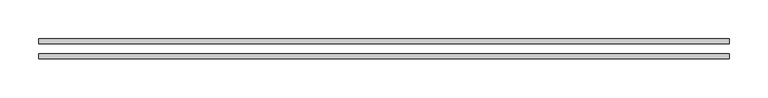
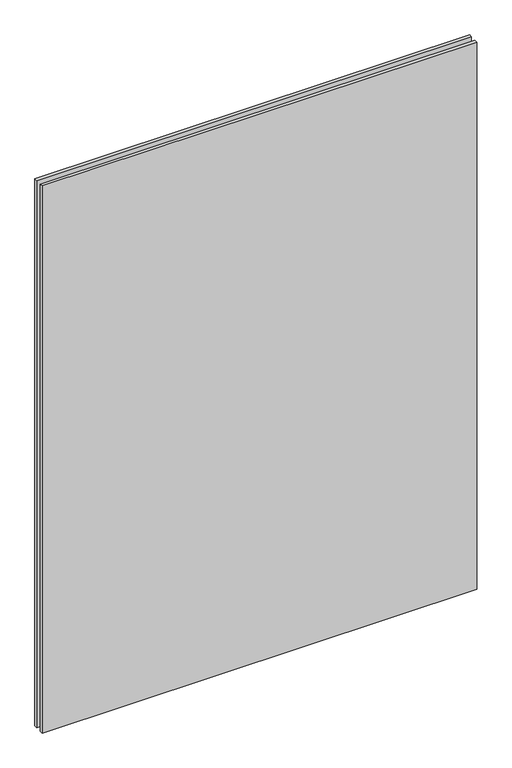
"""IFC4 building model written with IfcOpenShell, lengths in millimetres: proxy geometry, Window glass:Window glass:1:Window glass:1 : Window glass:Window glass:300352:337881:Window glass:1:Window glass:1 : Window glass:Window glass:300352:337881 : Window glass:Window glass:1:Window glass:1 : Window glass:Window glass:300352:337881:1 : Window glass:Window glass:1:Window glass:1 : Window glass:Window glass:300352:337881:Window glass:1:Window glass:1 : Window glass:Window glass:300352:337881 : Window glass:Window glass:1:Window glass:1 : Window glass:Window glass:300352:337881:301362."""

from ifc_helpers import new_model, si_unit, frame, origin, place, context, project, spatial, polyline, outline, extrude, source, transform, mapped, element, save


def generic_models_0ff10017(model_context):
    return source(origin(), model_context, "Body", "SweptSolid", [
        extrude(outline(polyline([(570404.7161787, -579048.3332724), (569517.4978941, -579048.3332724), (569517.4978941, -579041.9832724), (570404.7161787, -579041.9832724), (570404.7161787, -579048.3332724)])), frame((0.0, 0.0, 2479.9705452), z_axis=(0.0, 0.0, 1.0), x_axis=(1.0, 0.0, 0.0)), (0.0, 0.0, 1.0), 1180.5089096),
        extrude(outline(polyline([(570404.7161787, -579029.2832724), (569517.4978941, -579029.2832724), (569517.4978941, -579022.9332724), (570404.7161787, -579022.9332724), (570404.7161787, -579029.2832724)])), frame((0.0, 0.0, 2479.9705452), z_axis=(0.0, 0.0, 1.0), x_axis=(1.0, 0.0, 0.0)), (0.0, 0.0, 1.0), 1180.5089096),
    ])


if __name__ == "__main__":
    model = new_model("IFC4")
    model_context = context("Model", 3, world=origin())
    ifc_project = project(units=[si_unit("LENGTHUNIT", "METRE", prefix="MILLI")], contexts=[model_context])
    site = spatial("IfcSite", under=ifc_project)
    building = spatial("IfcBuilding", under=site)
    placement = place(None, origin())
    generic_models_shape = generic_models_0ff10017(model_context)
    element("IfcBuildingElementProxy", 1, Name="Window glass:Window glass:1:Window glass:1 : Window glass:Window glass:300352:337881:Window glass:1:Window glass:1 : Window glass:Window glass:300352:337881 : Window glass:Window glass:1:Window glass:1 : Window glass:Window glass:300352:337881:1 : Window glass:Window glass:1:Window glass:1 : Window glass:Window glass:300352:337881:Window glass:1:Window glass:1 : Window glass:Window glass:300352:337881 : Window glass:Window glass:1:Window glass:1 : Window glass:Window glass:300352:337881:301362", ObjectType="Window glass:Window glass:1:Window glass:1 : Window glass:Window glass:300352:337881:Window glass:1:Window glass:1 : Window glass:Window glass:300352:337881 : Window glass:Window glass:1:Window glass:1 : Window glass:Window glass:300352:337881:1 : Window glass:Window glass:1:Window glass:1 : Window glass:Window glass:300352:337881:Window glass:1:Window glass:1 : Window glass:Window glass:300352:337881 : Window glass:Window glass:1:Window glass:1 : Window glass:Window glass:300352:337881:301362", at=placement, inside=building, context=model_context, shape_type="MappedRepresentation", body=[
        mapped(generic_models_shape, transform((0.0, 0.0, 0.0), x_axis=(1.0, 0.0, 0.0), y_axis=(0.0, 1.0, 0.0), z_axis=(0.0, 0.0, 1.0))),
    ])
    save(model, "model.ifc")

# Revit data of these elements
# Type "Window glass:Window glass:1:Window glass:1 : Window glass:Window glass:300352:337881:Window glass:1:Window glass:1 : Window glass:Window glass:300352:337881 : Window glass:Window glass:1:Window glass:1 : Window glass:Window glass:300352:337881:1 : Window glass:Window glass:1:Window glass:1 : Window glass:Window glass:300352:337881:Window glass:1:Window glass:1 : Window glass:Window glass:300352:337881 : Window glass:Window glass:1:Window glass:1 : Window glass:Window glass:300352:337881:301362"
#   NameOverride = "Window glass:Window glass:1:Window glass:1 : Window glass:Window glass:300352:337881:Window glass:1:Window glass:1 : Window glass:Window glass:300352:337881 : Window glass:Window glass:1:Window glass:1 : Window glass:Window glass:300352:337881:301362"
#   ObjectTypeOverride = "Window glass:1:Window glass:1 : Window glass:Window glass:300352:337881 : Window glass:Window glass:1:Window glass:1 : Window glass:Window glass:300352:337881"
#   Reference = "Window glass"
#   Tag = "301362"
# Element 1 (IfcBuildingElementProxy, "Window glass:Window glass:1:Window glass:1 : Window glass:Window glass:300352:337881:Window glass:1:Window glass:1 : Window glass:Window glass:300352:337881 : Window glass:Window glass:1:Window glass:1 : Window glass:Window glass:300352:337881:1 : Window glass:Window glass:1:Window glass:1 : Window glass:Window glass:300352:337881:Window glass:1:Window glass:1 : Window glass:Window glass:300352:337881 : Window glass:Window glass:1:Window glass:1 : Window glass:Window glass:300352:337881:301362")
#   Materials on its faces: "INSULATED LOW-E GLAZING (SEE ELEVATIONS FOR U-FACTOR, SHGC, & LT)"
# Materials
#   "INSULATED LOW-E GLAZING (SEE ELEVATIONS FOR U-FACTOR, SHGC, & LT)": class "Unassigned", colour RGB 84 171 255, transparency 0, Cost = 0
